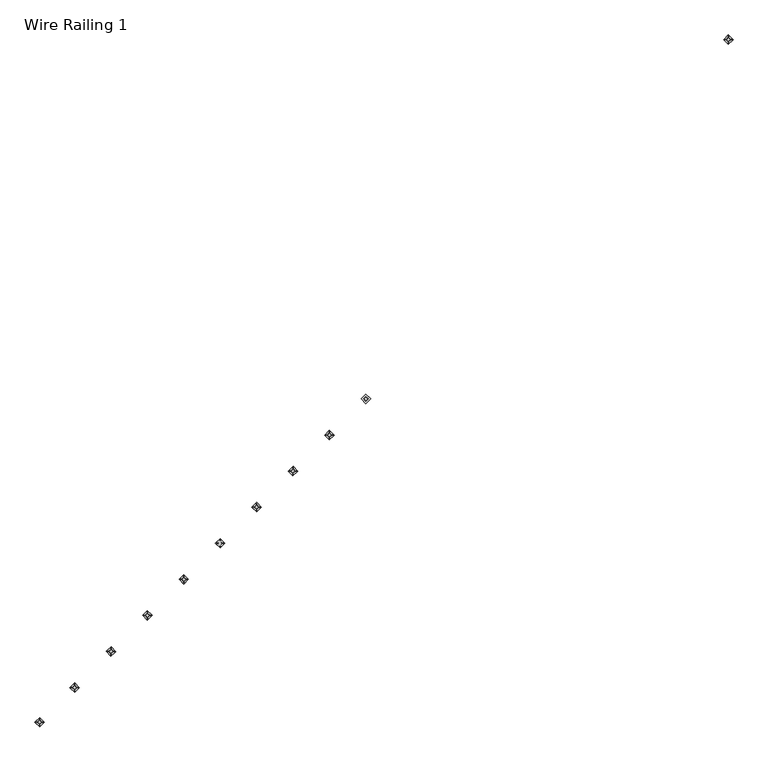
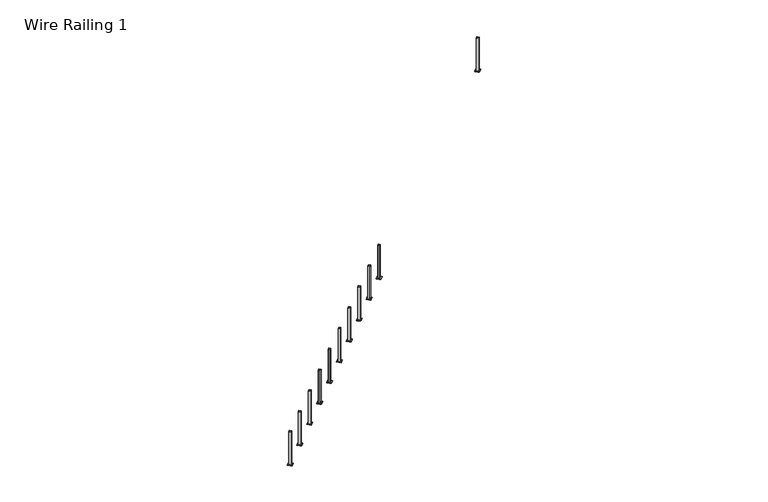
"""IFC4 building model written with IfcOpenShell, lengths in millimetres: railing geometry, Wire Railing 1."""

from ifc_helpers import new_model, si_unit, point, frame, frame_2d, origin, place, context, project, spatial, polyline, circle_curve, trimmed, segment, composite_curve, outline, extrude, source, transform, mapped, element, save


def wire_railing_1_c849696a(model_context):
    return source(origin(), model_context, "Body", "SweptSolid", [
        extrude(outline(polyline([(38725.9551823, 30541.0321501), (38816.1604279, 30630.430213), (38905.5584909, 30540.2249673), (38815.3532452, 30450.8269044), (38725.9551823, 30541.0321501)])), frame((0.0, 0.0, 263956.8), z_axis=(0.0, 0.0, 1.0), x_axis=(1.0, 0.0, 0.0)), (0.0, 0.0, 1.0), 6.35),
        extrude(outline(polyline([(38773.1010508, 30540.8202646), (38815.9485425, 30583.2843445), (38858.4126224, 30540.4368528), (38815.5651307, 30497.9727729), (38773.1010508, 30540.8202646)]), holes=[polyline([(38782.0812162, 30540.7799055), (38815.6054898, 30506.9529383), (38849.4324569, 30540.4772119), (38815.9081833, 30574.3041791), (38782.0812162, 30540.7799055)])]), frame((0.0, 0.0, 263956.8), z_axis=(0.0, 0.0, 1.0), x_axis=(1.0, 0.0, 0.0)), (0.0, 0.0, 1.0), 1047.75),
        extrude(outline(composite_curve([segment(trimmed(circle_curve(frame_2d((38120.0580506, 29788.5739154)), 6.35), [point((38124.5279538, 29784.0636531))], [point((38115.5881475, 29793.0841776))], False, "CARTESIAN"), True, "CONTINUOUS"), segment(trimmed(circle_curve(frame_2d((38120.0580506, 29788.5739154)), 6.35), [point((38115.5881475, 29793.0841776))], [point((38124.5279538, 29784.0636531))], False, "CARTESIAN"), True, "CONTINUOUS")], self_intersect=False)), frame((0.0, 0.0, 263956.8), z_axis=(0.0, 0.0, 1.0), x_axis=(1.0, 0.0, 0.0)), (0.0, 0.0, 1.0), 12.7),
        extrude(outline(composite_curve([segment(trimmed(circle_curve(frame_2d((38057.4794066, 29851.7175873)), 6.35), [point((38061.9493097, 29847.207325))], [point((38053.0095034, 29856.2278496))], False, "CARTESIAN"), True, "CONTINUOUS"), segment(trimmed(circle_curve(frame_2d((38057.4794066, 29851.7175873)), 6.35), [point((38053.0095034, 29856.2278496))], [point((38061.9493097, 29847.207325))], False, "CARTESIAN"), True, "CONTINUOUS")], self_intersect=False)), frame((0.0, 0.0, 263956.8), z_axis=(0.0, 0.0, 1.0), x_axis=(1.0, 0.0, 0.0)), (0.0, 0.0, 1.0), 12.7),
        extrude(outline(composite_curve([segment(trimmed(circle_curve(frame_2d((38183.2017226, 29851.1525594)), 6.35), [point((38187.6716257, 29846.6422971))], [point((38178.7318194, 29855.6628217))], False, "CARTESIAN"), True, "CONTINUOUS"), segment(trimmed(circle_curve(frame_2d((38183.2017226, 29851.1525594)), 6.35), [point((38178.7318194, 29855.6628217))], [point((38187.6716257, 29846.6422971))], False, "CARTESIAN"), True, "CONTINUOUS")], self_intersect=False)), frame((0.0, 0.0, 263956.8), z_axis=(0.0, 0.0, 1.0), x_axis=(1.0, 0.0, 0.0)), (0.0, 0.0, 1.0), 12.7),
        extrude(outline(composite_curve([segment(trimmed(circle_curve(frame_2d((38120.6230785, 29914.2962314)), 6.35), [point((38125.0929817, 29909.7859691))], [point((38116.1531754, 29918.8064936))], False, "CARTESIAN"), True, "CONTINUOUS"), segment(trimmed(circle_curve(frame_2d((38120.6230785, 29914.2962314)), 6.35), [point((38116.1531754, 29918.8064936))], [point((38125.0929817, 29909.7859691))], False, "CARTESIAN"), True, "CONTINUOUS")], self_intersect=False)), frame((0.0, 0.0, 263956.8), z_axis=(0.0, 0.0, 1.0), x_axis=(1.0, 0.0, 0.0)), (0.0, 0.0, 1.0), 12.7),
        extrude(outline(polyline([(38030.5389103, 29851.8386647), (38120.7441559, 29941.2367277), (38210.1422189, 29851.031482), (38119.9369732, 29761.6334191), (38030.5389103, 29851.8386647)])), frame((0.0, 0.0, 263956.8), z_axis=(0.0, 0.0, 1.0), x_axis=(1.0, 0.0, 0.0)), (0.0, 0.0, 1.0), 6.35),
        extrude(outline(polyline([(38077.6847788, 29851.6267793), (38120.5322705, 29894.0908591), (38162.9963504, 29851.2433675), (38120.1488587, 29808.7792876), (38077.6847788, 29851.6267793)]), holes=[polyline([(38086.6649442, 29851.5864201), (38120.1892178, 29817.759453), (38154.0161849, 29851.2837266), (38120.4919113, 29885.1106937), (38086.6649442, 29851.5864201)])]), frame((0.0, 0.0, 263956.8), z_axis=(0.0, 0.0, 1.0), x_axis=(1.0, 0.0, 0.0)), (0.0, 0.0, 1.0), 1047.75),
        extrude(outline(composite_curve([segment(trimmed(circle_curve(frame_2d((37424.6417786, 29099.38043)), 6.35), [point((37429.1116818, 29094.8701677))], [point((37420.1718755, 29103.8906923))], False, "CARTESIAN"), True, "CONTINUOUS"), segment(trimmed(circle_curve(frame_2d((37424.6417786, 29099.38043)), 6.35), [point((37420.1718755, 29103.8906923))], [point((37429.1116818, 29094.8701677))], False, "CARTESIAN"), True, "CONTINUOUS")], self_intersect=False)), frame((0.0, 0.0, 263956.8), z_axis=(0.0, 0.0, 1.0), x_axis=(1.0, 0.0, 0.0)), (0.0, 0.0, 1.0), 12.7),
        extrude(outline(composite_curve([segment(trimmed(circle_curve(frame_2d((37362.0631346, 29162.524102)), 6.35), [point((37366.5330377, 29158.0138397))], [point((37357.5932314, 29167.0343643))], False, "CARTESIAN"), True, "CONTINUOUS"), segment(trimmed(circle_curve(frame_2d((37362.0631346, 29162.524102)), 6.35), [point((37357.5932314, 29167.0343643))], [point((37366.5330377, 29158.0138397))], False, "CARTESIAN"), True, "CONTINUOUS")], self_intersect=False)), frame((0.0, 0.0, 263956.8), z_axis=(0.0, 0.0, 1.0), x_axis=(1.0, 0.0, 0.0)), (0.0, 0.0, 1.0), 12.7),
        extrude(outline(composite_curve([segment(trimmed(circle_curve(frame_2d((37487.7854506, 29161.9590741)), 6.35), [point((37492.2553537, 29157.4488118))], [point((37483.3155474, 29166.4693364))], False, "CARTESIAN"), True, "CONTINUOUS"), segment(trimmed(circle_curve(frame_2d((37487.7854506, 29161.9590741)), 6.35), [point((37483.3155474, 29166.4693364))], [point((37492.2553537, 29157.4488118))], False, "CARTESIAN"), True, "CONTINUOUS")], self_intersect=False)), frame((0.0, 0.0, 263956.8), z_axis=(0.0, 0.0, 1.0), x_axis=(1.0, 0.0, 0.0)), (0.0, 0.0, 1.0), 12.7),
        extrude(outline(composite_curve([segment(trimmed(circle_curve(frame_2d((37425.2068065, 29225.102746)), 6.35), [point((37429.6767097, 29220.5924837))], [point((37420.7369034, 29229.6130083))], False, "CARTESIAN"), True, "CONTINUOUS"), segment(trimmed(circle_curve(frame_2d((37425.2068065, 29225.102746)), 6.35), [point((37420.7369034, 29229.6130083))], [point((37429.6767097, 29220.5924837))], False, "CARTESIAN"), True, "CONTINUOUS")], self_intersect=False)), frame((0.0, 0.0, 263956.8), z_axis=(0.0, 0.0, 1.0), x_axis=(1.0, 0.0, 0.0)), (0.0, 0.0, 1.0), 12.7),
        extrude(outline(polyline([(37335.1226383, 29162.6451794), (37425.3278839, 29252.0432423), (37514.7259469, 29161.8379967), (37424.5207012, 29072.4399337), (37335.1226383, 29162.6451794)])), frame((0.0, 0.0, 263956.8), z_axis=(0.0, 0.0, 1.0), x_axis=(1.0, 0.0, 0.0)), (0.0, 0.0, 1.0), 6.35),
        extrude(outline(polyline([(37382.2685068, 29162.4332939), (37425.1159985, 29204.8973738), (37467.5800784, 29162.0498821), (37424.7325867, 29119.5858022), (37382.2685068, 29162.4332939)]), holes=[polyline([(37391.2486722, 29162.3929348), (37424.7729458, 29128.5659677), (37458.5999129, 29162.0902413), (37425.0756393, 29195.9172084), (37391.2486722, 29162.3929348)])]), frame((0.0, 0.0, 263956.8), z_axis=(0.0, 0.0, 1.0), x_axis=(1.0, 0.0, 0.0)), (0.0, 0.0, 1.0), 1047.75),
        extrude(outline(composite_curve([segment(trimmed(circle_curve(frame_2d((36729.2255066, 28410.1869447)), 6.35), [point((36733.6954098, 28405.6766824))], [point((36724.7556035, 28414.697207))], False, "CARTESIAN"), True, "CONTINUOUS"), segment(trimmed(circle_curve(frame_2d((36729.2255066, 28410.1869447)), 6.35), [point((36724.7556035, 28414.697207))], [point((36733.6954098, 28405.6766824))], False, "CARTESIAN"), True, "CONTINUOUS")], self_intersect=False)), frame((0.0, 0.0, 263956.8), z_axis=(0.0, 0.0, 1.0), x_axis=(1.0, 0.0, 0.0)), (0.0, 0.0, 1.0), 12.7),
        extrude(outline(composite_curve([segment(trimmed(circle_curve(frame_2d((36666.6468626, 28473.3306166)), 6.35), [point((36671.1167657, 28468.8203544))], [point((36662.1769594, 28477.8408789))], False, "CARTESIAN"), True, "CONTINUOUS"), segment(trimmed(circle_curve(frame_2d((36666.6468626, 28473.3306166)), 6.35), [point((36662.1769594, 28477.8408789))], [point((36671.1167657, 28468.8203544))], False, "CARTESIAN"), True, "CONTINUOUS")], self_intersect=False)), frame((0.0, 0.0, 263956.8), z_axis=(0.0, 0.0, 1.0), x_axis=(1.0, 0.0, 0.0)), (0.0, 0.0, 1.0), 12.7),
        extrude(outline(composite_curve([segment(trimmed(circle_curve(frame_2d((36792.3691786, 28472.7655887)), 6.35), [point((36796.8390817, 28468.2553265))], [point((36787.8992754, 28477.275851))], False, "CARTESIAN"), True, "CONTINUOUS"), segment(trimmed(circle_curve(frame_2d((36792.3691786, 28472.7655887)), 6.35), [point((36787.8992754, 28477.275851))], [point((36796.8390817, 28468.2553265))], False, "CARTESIAN"), True, "CONTINUOUS")], self_intersect=False)), frame((0.0, 0.0, 263956.8), z_axis=(0.0, 0.0, 1.0), x_axis=(1.0, 0.0, 0.0)), (0.0, 0.0, 1.0), 12.7),
        extrude(outline(composite_curve([segment(trimmed(circle_curve(frame_2d((36729.7905345, 28535.9092607)), 6.35), [point((36734.2604377, 28531.3989984))], [point((36725.3206314, 28540.419523))], False, "CARTESIAN"), True, "CONTINUOUS"), segment(trimmed(circle_curve(frame_2d((36729.7905345, 28535.9092607)), 6.35), [point((36725.3206314, 28540.419523))], [point((36734.2604377, 28531.3989984))], False, "CARTESIAN"), True, "CONTINUOUS")], self_intersect=False)), frame((0.0, 0.0, 263956.8), z_axis=(0.0, 0.0, 1.0), x_axis=(1.0, 0.0, 0.0)), (0.0, 0.0, 1.0), 12.7),
        extrude(outline(polyline([(36639.7063663, 28473.4516941), (36729.9116119, 28562.849757), (36819.3096749, 28472.6445113), (36729.1044292, 28383.2464484), (36639.7063663, 28473.4516941)])), frame((0.0, 0.0, 263956.8), z_axis=(0.0, 0.0, 1.0), x_axis=(1.0, 0.0, 0.0)), (0.0, 0.0, 1.0), 6.35),
        extrude(outline(polyline([(36686.8522348, 28473.2398086), (36729.6997265, 28515.7038885), (36772.1638064, 28472.8563968), (36729.3163147, 28430.3923169), (36686.8522348, 28473.2398086)]), holes=[polyline([(36695.8324002, 28473.1994495), (36729.3566738, 28439.3724823), (36763.1836409, 28472.8967559), (36729.6593673, 28506.7237231), (36695.8324002, 28473.1994495)])]), frame((0.0, 0.0, 263956.8), z_axis=(0.0, 0.0, 1.0), x_axis=(1.0, 0.0, 0.0)), (0.0, 0.0, 1.0), 1047.75),
        extrude(outline(composite_curve([segment(trimmed(circle_curve(frame_2d((36033.8092346, 27720.9934594)), 6.35), [point((36038.2791378, 27716.4831971))], [point((36029.3393315, 27725.5037216))], False, "CARTESIAN"), True, "CONTINUOUS"), segment(trimmed(circle_curve(frame_2d((36033.8092346, 27720.9934594)), 6.35), [point((36029.3393315, 27725.5037216))], [point((36038.2791378, 27716.4831971))], False, "CARTESIAN"), True, "CONTINUOUS")], self_intersect=False)), frame((0.0, 0.0, 263956.8), z_axis=(0.0, 0.0, 1.0), x_axis=(1.0, 0.0, 0.0)), (0.0, 0.0, 1.0), 12.7),
        extrude(outline(composite_curve([segment(trimmed(circle_curve(frame_2d((35971.2305906, 27784.1371313)), 6.35), [point((35975.7004937, 27779.626869))], [point((35966.7606874, 27788.6473936))], False, "CARTESIAN"), True, "CONTINUOUS"), segment(trimmed(circle_curve(frame_2d((35971.2305906, 27784.1371313)), 6.35), [point((35966.7606874, 27788.6473936))], [point((35975.7004937, 27779.626869))], False, "CARTESIAN"), True, "CONTINUOUS")], self_intersect=False)), frame((0.0, 0.0, 263956.8), z_axis=(0.0, 0.0, 1.0), x_axis=(1.0, 0.0, 0.0)), (0.0, 0.0, 1.0), 12.7),
        extrude(outline(composite_curve([segment(trimmed(circle_curve(frame_2d((36096.9529066, 27783.5721034)), 6.35), [point((36101.4228097, 27779.0618411))], [point((36092.4830034, 27788.0823657))], False, "CARTESIAN"), True, "CONTINUOUS"), segment(trimmed(circle_curve(frame_2d((36096.9529066, 27783.5721034)), 6.35), [point((36092.4830034, 27788.0823657))], [point((36101.4228097, 27779.0618411))], False, "CARTESIAN"), True, "CONTINUOUS")], self_intersect=False)), frame((0.0, 0.0, 263956.8), z_axis=(0.0, 0.0, 1.0), x_axis=(1.0, 0.0, 0.0)), (0.0, 0.0, 1.0), 12.7),
        extrude(outline(composite_curve([segment(trimmed(circle_curve(frame_2d((36034.3742625, 27846.7157754)), 6.35), [point((36038.8441657, 27842.2055131))], [point((36029.9043594, 27851.2260376))], False, "CARTESIAN"), True, "CONTINUOUS"), segment(trimmed(circle_curve(frame_2d((36034.3742625, 27846.7157754)), 6.35), [point((36029.9043594, 27851.2260376))], [point((36038.8441657, 27842.2055131))], False, "CARTESIAN"), True, "CONTINUOUS")], self_intersect=False)), frame((0.0, 0.0, 263956.8), z_axis=(0.0, 0.0, 1.0), x_axis=(1.0, 0.0, 0.0)), (0.0, 0.0, 1.0), 12.7),
        extrude(outline(polyline([(35944.2900943, 27784.2582087), (36034.4953399, 27873.6562717), (36123.8934029, 27783.451026), (36033.6881572, 27694.0529631), (35944.2900943, 27784.2582087)])), frame((0.0, 0.0, 263956.8), z_axis=(0.0, 0.0, 1.0), x_axis=(1.0, 0.0, 0.0)), (0.0, 0.0, 1.0), 6.35),
        extrude(outline(polyline([(35991.4359628, 27784.0463233), (36034.2834545, 27826.5104031), (36076.7475344, 27783.6629115), (36033.9000427, 27741.1988316), (35991.4359628, 27784.0463233)]), holes=[polyline([(36000.4161282, 27784.0059641), (36033.9404018, 27750.178997), (36067.7673689, 27783.7032706), (36034.2430953, 27817.5302377), (36000.4161282, 27784.0059641)])]), frame((0.0, 0.0, 263956.8), z_axis=(0.0, 0.0, 1.0), x_axis=(1.0, 0.0, 0.0)), (0.0, 0.0, 1.0), 1047.75),
        extrude(outline(composite_curve([segment(trimmed(circle_curve(frame_2d((35338.3929626, 27031.799974)), 6.35), [point((35342.8628658, 27027.2897117))], [point((35333.9230595, 27036.3102363))], False, "CARTESIAN"), True, "CONTINUOUS"), segment(trimmed(circle_curve(frame_2d((35338.3929626, 27031.799974)), 6.35), [point((35333.9230595, 27036.3102363))], [point((35342.8628658, 27027.2897117))], False, "CARTESIAN"), True, "CONTINUOUS")], self_intersect=False)), frame((0.0, 0.0, 263956.8), z_axis=(0.0, 0.0, 1.0), x_axis=(1.0, 0.0, 0.0)), (0.0, 0.0, 1.0), 12.7),
        extrude(outline(composite_curve([segment(trimmed(circle_curve(frame_2d((35275.8143186, 27094.943646)), 6.35), [point((35280.2842217, 27090.4333837))], [point((35271.3444154, 27099.4539083))], False, "CARTESIAN"), True, "CONTINUOUS"), segment(trimmed(circle_curve(frame_2d((35275.8143186, 27094.943646)), 6.35), [point((35271.3444154, 27099.4539083))], [point((35280.2842217, 27090.4333837))], False, "CARTESIAN"), True, "CONTINUOUS")], self_intersect=False)), frame((0.0, 0.0, 263956.8), z_axis=(0.0, 0.0, 1.0), x_axis=(1.0, 0.0, 0.0)), (0.0, 0.0, 1.0), 12.7),
        extrude(outline(composite_curve([segment(trimmed(circle_curve(frame_2d((35401.5366346, 27094.3786181)), 6.35), [point((35406.0065377, 27089.8683558))], [point((35397.0667314, 27098.8888804))], False, "CARTESIAN"), True, "CONTINUOUS"), segment(trimmed(circle_curve(frame_2d((35401.5366346, 27094.3786181)), 6.35), [point((35397.0667314, 27098.8888804))], [point((35406.0065377, 27089.8683558))], False, "CARTESIAN"), True, "CONTINUOUS")], self_intersect=False)), frame((0.0, 0.0, 263956.8), z_axis=(0.0, 0.0, 1.0), x_axis=(1.0, 0.0, 0.0)), (0.0, 0.0, 1.0), 12.7),
        extrude(outline(composite_curve([segment(trimmed(circle_curve(frame_2d((35338.9579905, 27157.52229)), 6.35), [point((35343.4278937, 27153.0120277))], [point((35334.4880874, 27162.0325523))], False, "CARTESIAN"), True, "CONTINUOUS"), segment(trimmed(circle_curve(frame_2d((35338.9579905, 27157.52229)), 6.35), [point((35334.4880874, 27162.0325523))], [point((35343.4278937, 27153.0120277))], False, "CARTESIAN"), True, "CONTINUOUS")], self_intersect=False)), frame((0.0, 0.0, 263956.8), z_axis=(0.0, 0.0, 1.0), x_axis=(1.0, 0.0, 0.0)), (0.0, 0.0, 1.0), 12.7),
        extrude(outline(polyline([(35248.8738223, 27095.0647234), (35339.0790679, 27184.4627863), (35428.4771309, 27094.2575407), (35338.2718852, 27004.8594777), (35248.8738223, 27095.0647234)])), frame((0.0, 0.0, 263956.8), z_axis=(0.0, 0.0, 1.0), x_axis=(1.0, 0.0, 0.0)), (0.0, 0.0, 1.0), 6.35),
        extrude(outline(polyline([(35296.0196908, 27094.8528379), (35338.8671825, 27137.3169178), (35381.3312624, 27094.4694261), (35338.4837707, 27052.0053462), (35296.0196908, 27094.8528379)]), holes=[polyline([(35304.9998562, 27094.8124788), (35338.5241298, 27060.9855117), (35372.3510969, 27094.5097853), (35338.8268233, 27128.3367524), (35304.9998562, 27094.8124788)])]), frame((0.0, 0.0, 263956.8), z_axis=(0.0, 0.0, 1.0), x_axis=(1.0, 0.0, 0.0)), (0.0, 0.0, 1.0), 1047.75),
        extrude(outline(composite_curve([segment(trimmed(circle_curve(frame_2d((34642.9766906, 26342.6064887)), 6.35), [point((34647.4465938, 26338.0962264))], [point((34638.5067875, 26347.116751))], False, "CARTESIAN"), True, "CONTINUOUS"), segment(trimmed(circle_curve(frame_2d((34642.9766906, 26342.6064887)), 6.35), [point((34638.5067875, 26347.116751))], [point((34647.4465938, 26338.0962264))], False, "CARTESIAN"), True, "CONTINUOUS")], self_intersect=False)), frame((0.0, 0.0, 263956.8), z_axis=(0.0, 0.0, 1.0), x_axis=(1.0, 0.0, 0.0)), (0.0, 0.0, 1.0), 12.7),
        extrude(outline(composite_curve([segment(trimmed(circle_curve(frame_2d((34580.3980466, 26405.7501606)), 6.35), [point((34584.8679497, 26401.2398984))], [point((34575.9281434, 26410.2604229))], False, "CARTESIAN"), True, "CONTINUOUS"), segment(trimmed(circle_curve(frame_2d((34580.3980466, 26405.7501606)), 6.35), [point((34575.9281434, 26410.2604229))], [point((34584.8679497, 26401.2398984))], False, "CARTESIAN"), True, "CONTINUOUS")], self_intersect=False)), frame((0.0, 0.0, 263956.8), z_axis=(0.0, 0.0, 1.0), x_axis=(1.0, 0.0, 0.0)), (0.0, 0.0, 1.0), 12.7),
        extrude(outline(composite_curve([segment(trimmed(circle_curve(frame_2d((34706.1203626, 26405.1851327)), 6.35), [point((34710.5902657, 26400.6748705))], [point((34701.6504594, 26409.695395))], False, "CARTESIAN"), True, "CONTINUOUS"), segment(trimmed(circle_curve(frame_2d((34706.1203626, 26405.1851327)), 6.35), [point((34701.6504594, 26409.695395))], [point((34710.5902657, 26400.6748705))], False, "CARTESIAN"), True, "CONTINUOUS")], self_intersect=False)), frame((0.0, 0.0, 263956.8), z_axis=(0.0, 0.0, 1.0), x_axis=(1.0, 0.0, 0.0)), (0.0, 0.0, 1.0), 12.7),
        extrude(outline(composite_curve([segment(trimmed(circle_curve(frame_2d((34643.5417185, 26468.3288047)), 6.35), [point((34648.0116217, 26463.8185424))], [point((34639.0718154, 26472.839067))], False, "CARTESIAN"), True, "CONTINUOUS"), segment(trimmed(circle_curve(frame_2d((34643.5417185, 26468.3288047)), 6.35), [point((34639.0718154, 26472.839067))], [point((34648.0116217, 26463.8185424))], False, "CARTESIAN"), True, "CONTINUOUS")], self_intersect=False)), frame((0.0, 0.0, 263956.8), z_axis=(0.0, 0.0, 1.0), x_axis=(1.0, 0.0, 0.0)), (0.0, 0.0, 1.0), 12.7),
        extrude(outline(polyline([(34553.4575503, 26405.8712381), (34643.6627959, 26495.269301), (34733.0608589, 26405.0640553), (34642.8556132, 26315.6659924), (34553.4575503, 26405.8712381)])), frame((0.0, 0.0, 263956.8), z_axis=(0.0, 0.0, 1.0), x_axis=(1.0, 0.0, 0.0)), (0.0, 0.0, 1.0), 6.35),
        extrude(outline(polyline([(34600.6034188, 26405.6593526), (34643.4509105, 26448.1234325), (34685.9149903, 26405.2759408), (34643.0674987, 26362.8118609), (34600.6034188, 26405.6593526)]), holes=[polyline([(34609.5835842, 26405.6189935), (34643.1078578, 26371.7920263), (34676.9348249, 26405.3162999), (34643.4105513, 26439.1432671), (34609.5835842, 26405.6189935)])]), frame((0.0, 0.0, 263956.8), z_axis=(0.0, 0.0, 1.0), x_axis=(1.0, 0.0, 0.0)), (0.0, 0.0, 1.0), 1047.75),
        extrude(outline(composite_curve([segment(trimmed(circle_curve(frame_2d((33947.5604186, 25653.4130034)), 6.35), [point((33952.0303217, 25648.9027411))], [point((33943.0905155, 25657.9232656))], False, "CARTESIAN"), True, "CONTINUOUS"), segment(trimmed(circle_curve(frame_2d((33947.5604186, 25653.4130034)), 6.35), [point((33943.0905155, 25657.9232656))], [point((33952.0303217, 25648.9027411))], False, "CARTESIAN"), True, "CONTINUOUS")], self_intersect=False)), frame((0.0, 0.0, 263956.8), z_axis=(0.0, 0.0, 1.0), x_axis=(1.0, 0.0, 0.0)), (0.0, 0.0, 1.0), 12.7),
        extrude(outline(composite_curve([segment(trimmed(circle_curve(frame_2d((33884.9817745, 25716.5566753)), 6.35), [point((33889.4516777, 25712.046413))], [point((33880.5118714, 25721.0669376))], False, "CARTESIAN"), True, "CONTINUOUS"), segment(trimmed(circle_curve(frame_2d((33884.9817745, 25716.5566753)), 6.35), [point((33880.5118714, 25721.0669376))], [point((33889.4516777, 25712.046413))], False, "CARTESIAN"), True, "CONTINUOUS")], self_intersect=False)), frame((0.0, 0.0, 263956.8), z_axis=(0.0, 0.0, 1.0), x_axis=(1.0, 0.0, 0.0)), (0.0, 0.0, 1.0), 12.7),
        extrude(outline(composite_curve([segment(trimmed(circle_curve(frame_2d((34010.7040906, 25715.9916474)), 6.35), [point((34015.1739937, 25711.4813851))], [point((34006.2341874, 25720.5019097))], False, "CARTESIAN"), True, "CONTINUOUS"), segment(trimmed(circle_curve(frame_2d((34010.7040906, 25715.9916474)), 6.35), [point((34006.2341874, 25720.5019097))], [point((34015.1739937, 25711.4813851))], False, "CARTESIAN"), True, "CONTINUOUS")], self_intersect=False)), frame((0.0, 0.0, 263956.8), z_axis=(0.0, 0.0, 1.0), x_axis=(1.0, 0.0, 0.0)), (0.0, 0.0, 1.0), 12.7),
        extrude(outline(composite_curve([segment(trimmed(circle_curve(frame_2d((33948.1254465, 25779.1353194)), 6.35), [point((33952.5953497, 25774.6250571))], [point((33943.6555434, 25783.6455816))], False, "CARTESIAN"), True, "CONTINUOUS"), segment(trimmed(circle_curve(frame_2d((33948.1254465, 25779.1353194)), 6.35), [point((33943.6555434, 25783.6455816))], [point((33952.5953497, 25774.6250571))], False, "CARTESIAN"), True, "CONTINUOUS")], self_intersect=False)), frame((0.0, 0.0, 263956.8), z_axis=(0.0, 0.0, 1.0), x_axis=(1.0, 0.0, 0.0)), (0.0, 0.0, 1.0), 12.7),
        extrude(outline(polyline([(33858.0412783, 25716.6777527), (33948.2465239, 25806.0758157), (34037.6445869, 25715.87057), (33947.4393412, 25626.4725071), (33858.0412783, 25716.6777527)])), frame((0.0, 0.0, 263956.8), z_axis=(0.0, 0.0, 1.0), x_axis=(1.0, 0.0, 0.0)), (0.0, 0.0, 1.0), 6.35),
        extrude(outline(polyline([(33905.1871468, 25716.4658673), (33948.0346385, 25758.9299472), (33990.4987183, 25716.0824555), (33947.6512267, 25673.6183756), (33905.1871468, 25716.4658673)]), holes=[polyline([(33914.1673122, 25716.4255081), (33947.6915858, 25682.598541), (33981.5185529, 25716.1228146), (33947.9942793, 25749.9497817), (33914.1673122, 25716.4255081)])]), frame((0.0, 0.0, 263956.8), z_axis=(0.0, 0.0, 1.0), x_axis=(1.0, 0.0, 0.0)), (0.0, 0.0, 1.0), 1047.75),
        extrude(outline(composite_curve([segment(trimmed(circle_curve(frame_2d((33252.1441466, 24964.219518)), 6.35), [point((33256.6140497, 24959.7092557))], [point((33247.6742435, 24968.7297803))], False, "CARTESIAN"), True, "CONTINUOUS"), segment(trimmed(circle_curve(frame_2d((33252.1441466, 24964.219518)), 6.35), [point((33247.6742435, 24968.7297803))], [point((33256.6140497, 24959.7092557))], False, "CARTESIAN"), True, "CONTINUOUS")], self_intersect=False)), frame((0.0, 0.0, 263956.8), z_axis=(0.0, 0.0, 1.0), x_axis=(1.0, 0.0, 0.0)), (0.0, 0.0, 1.0), 12.7),
        extrude(outline(composite_curve([segment(trimmed(circle_curve(frame_2d((33189.5655025, 25027.36319)), 6.35), [point((33194.0354057, 25022.8529277))], [point((33185.0955994, 25031.8734523))], False, "CARTESIAN"), True, "CONTINUOUS"), segment(trimmed(circle_curve(frame_2d((33189.5655025, 25027.36319)), 6.35), [point((33185.0955994, 25031.8734523))], [point((33194.0354057, 25022.8529277))], False, "CARTESIAN"), True, "CONTINUOUS")], self_intersect=False)), frame((0.0, 0.0, 263956.8), z_axis=(0.0, 0.0, 1.0), x_axis=(1.0, 0.0, 0.0)), (0.0, 0.0, 1.0), 12.7),
        extrude(outline(composite_curve([segment(trimmed(circle_curve(frame_2d((33315.2878186, 25026.7981621)), 6.35), [point((33319.7577217, 25022.2878998))], [point((33310.8179154, 25031.3084244))], False, "CARTESIAN"), True, "CONTINUOUS"), segment(trimmed(circle_curve(frame_2d((33315.2878186, 25026.7981621)), 6.35), [point((33310.8179154, 25031.3084244))], [point((33319.7577217, 25022.2878998))], False, "CARTESIAN"), True, "CONTINUOUS")], self_intersect=False)), frame((0.0, 0.0, 263956.8), z_axis=(0.0, 0.0, 1.0), x_axis=(1.0, 0.0, 0.0)), (0.0, 0.0, 1.0), 12.7),
        extrude(outline(composite_curve([segment(trimmed(circle_curve(frame_2d((33252.7091745, 25089.941834)), 6.35), [point((33257.1790777, 25085.4315718))], [point((33248.2392714, 25094.4520963))], False, "CARTESIAN"), True, "CONTINUOUS"), segment(trimmed(circle_curve(frame_2d((33252.7091745, 25089.941834)), 6.35), [point((33248.2392714, 25094.4520963))], [point((33257.1790777, 25085.4315718))], False, "CARTESIAN"), True, "CONTINUOUS")], self_intersect=False)), frame((0.0, 0.0, 263956.8), z_axis=(0.0, 0.0, 1.0), x_axis=(1.0, 0.0, 0.0)), (0.0, 0.0, 1.0), 12.7),
        extrude(outline(polyline([(33162.6250063, 25027.4842674), (33252.8302519, 25116.8823303), (33342.2283148, 25026.6770847), (33252.0230692, 24937.2790217), (33162.6250063, 25027.4842674)])), frame((0.0, 0.0, 263956.8), z_axis=(0.0, 0.0, 1.0), x_axis=(1.0, 0.0, 0.0)), (0.0, 0.0, 1.0), 6.35),
        extrude(outline(polyline([(33209.7708748, 25027.2723819), (33252.6183664, 25069.7364618), (33295.0824463, 25026.8889701), (33252.2349547, 24984.4248902), (33209.7708748, 25027.2723819)]), holes=[polyline([(33218.7510402, 25027.2320228), (33252.2753138, 24993.4050557), (33286.1022809, 25026.9293293), (33252.5780073, 25060.7562964), (33218.7510402, 25027.2320228)])]), frame((0.0, 0.0, 263956.8), z_axis=(0.0, 0.0, 1.0), x_axis=(1.0, 0.0, 0.0)), (0.0, 0.0, 1.0), 1047.75),
        extrude(outline(composite_curve([segment(trimmed(circle_curve(frame_2d((45742.575469, 37342.8828351)), 6.35), [point((45747.0453721, 37338.3725729))], [point((45738.1055658, 37347.3930974))], False, "CARTESIAN"), True, "CONTINUOUS"), segment(trimmed(circle_curve(frame_2d((45742.575469, 37342.8828351)), 6.35), [point((45738.1055658, 37347.3930974))], [point((45747.0453721, 37338.3725729))], False, "CARTESIAN"), True, "CONTINUOUS")], self_intersect=False)), frame((0.0, 0.0, 263956.8), z_axis=(0.0, 0.0, 1.0), x_axis=(1.0, 0.0, 0.0)), (0.0, 0.0, 1.0), 12.7),
        extrude(outline(composite_curve([segment(trimmed(circle_curve(frame_2d((45679.9968249, 37406.0265071)), 6.35), [point((45684.466728, 37401.5162448))], [point((45675.5269218, 37410.5367694))], False, "CARTESIAN"), True, "CONTINUOUS"), segment(trimmed(circle_curve(frame_2d((45679.9968249, 37406.0265071)), 6.35), [point((45675.5269218, 37410.5367694))], [point((45684.466728, 37401.5162448))], False, "CARTESIAN"), True, "CONTINUOUS")], self_intersect=False)), frame((0.0, 0.0, 263956.8), z_axis=(0.0, 0.0, 1.0), x_axis=(1.0, 0.0, 0.0)), (0.0, 0.0, 1.0), 12.7),
        extrude(outline(composite_curve([segment(trimmed(circle_curve(frame_2d((45805.7191409, 37405.4614792)), 6.35), [point((45810.1890441, 37400.9512169))], [point((45801.2492378, 37409.9717415))], False, "CARTESIAN"), True, "CONTINUOUS"), segment(trimmed(circle_curve(frame_2d((45805.7191409, 37405.4614792)), 6.35), [point((45801.2492378, 37409.9717415))], [point((45810.1890441, 37400.9512169))], False, "CARTESIAN"), True, "CONTINUOUS")], self_intersect=False)), frame((0.0, 0.0, 263956.8), z_axis=(0.0, 0.0, 1.0), x_axis=(1.0, 0.0, 0.0)), (0.0, 0.0, 1.0), 12.7),
        extrude(outline(composite_curve([segment(trimmed(circle_curve(frame_2d((45743.1404969, 37468.6051512)), 6.35), [point((45747.6104, 37464.0948889))], [point((45738.6705937, 37473.1154134))], False, "CARTESIAN"), True, "CONTINUOUS"), segment(trimmed(circle_curve(frame_2d((45743.1404969, 37468.6051512)), 6.35), [point((45738.6705937, 37473.1154134))], [point((45747.6104, 37464.0948889))], False, "CARTESIAN"), True, "CONTINUOUS")], self_intersect=False)), frame((0.0, 0.0, 263956.8), z_axis=(0.0, 0.0, 1.0), x_axis=(1.0, 0.0, 0.0)), (0.0, 0.0, 1.0), 12.7),
        extrude(outline(polyline([(45653.0563286, 37406.1475845), (45743.2615743, 37495.5456474), (45832.6596372, 37405.3404018), (45742.4543915, 37315.9423388), (45653.0563286, 37406.1475845)])), frame((0.0, 0.0, 263956.8), z_axis=(0.0, 0.0, 1.0), x_axis=(1.0, 0.0, 0.0)), (0.0, 0.0, 1.0), 6.35),
        extrude(outline(polyline([(45700.2021971, 37405.935699), (45743.0496888, 37448.3997789), (45785.5137687, 37405.5522872), (45742.666277, 37363.0882074), (45700.2021971, 37405.935699)]), holes=[polyline([(45709.1823625, 37405.8953399), (45742.7066361, 37372.0683728), (45776.5336033, 37405.5926464), (45743.0093297, 37439.4196135), (45709.1823625, 37405.8953399)])]), frame((0.0, 0.0, 263956.8), z_axis=(0.0, 0.0, 1.0), x_axis=(1.0, 0.0, 0.0)), (0.0, 0.0, 1.0), 1047.75),
        extrude(outline(composite_curve([segment(trimmed(circle_curve(frame_2d((32583.7894483, 24301.8454516)), 6.35), [point((32588.2593514, 24297.3351893))], [point((32579.3195451, 24306.3557139))], False, "CARTESIAN"), True, "CONTINUOUS"), segment(trimmed(circle_curve(frame_2d((32583.7894483, 24301.8454516)), 6.35), [point((32579.3195451, 24306.3557139))], [point((32588.2593514, 24297.3351893))], False, "CARTESIAN"), True, "CONTINUOUS")], self_intersect=False)), frame((0.0, 0.0, 263956.8), z_axis=(0.0, 0.0, 1.0), x_axis=(1.0, 0.0, 0.0)), (0.0, 0.0, 1.0), 12.7),
        extrude(outline(composite_curve([segment(trimmed(circle_curve(frame_2d((32521.2108042, 24364.9891235)), 6.35), [point((32525.6807074, 24360.4788612))], [point((32516.7409011, 24369.4993858))], False, "CARTESIAN"), True, "CONTINUOUS"), segment(trimmed(circle_curve(frame_2d((32521.2108042, 24364.9891235)), 6.35), [point((32516.7409011, 24369.4993858))], [point((32525.6807074, 24360.4788612))], False, "CARTESIAN"), True, "CONTINUOUS")], self_intersect=False)), frame((0.0, 0.0, 263956.8), z_axis=(0.0, 0.0, 1.0), x_axis=(1.0, 0.0, 0.0)), (0.0, 0.0, 1.0), 12.7),
        extrude(outline(composite_curve([segment(trimmed(circle_curve(frame_2d((32646.9331203, 24364.4240956)), 6.35), [point((32651.4030234, 24359.9138333))], [point((32642.4632171, 24368.9343579))], False, "CARTESIAN"), True, "CONTINUOUS"), segment(trimmed(circle_curve(frame_2d((32646.9331203, 24364.4240956)), 6.35), [point((32642.4632171, 24368.9343579))], [point((32651.4030234, 24359.9138333))], False, "CARTESIAN"), True, "CONTINUOUS")], self_intersect=False)), frame((0.0, 0.0, 263956.8), z_axis=(0.0, 0.0, 1.0), x_axis=(1.0, 0.0, 0.0)), (0.0, 0.0, 1.0), 12.7),
        extrude(outline(composite_curve([segment(trimmed(circle_curve(frame_2d((32584.3544762, 24427.5677676)), 6.35), [point((32588.8243793, 24423.0575053))], [point((32579.8845731, 24432.0780299))], False, "CARTESIAN"), True, "CONTINUOUS"), segment(trimmed(circle_curve(frame_2d((32584.3544762, 24427.5677676)), 6.35), [point((32579.8845731, 24432.0780299))], [point((32588.8243793, 24423.0575053))], False, "CARTESIAN"), True, "CONTINUOUS")], self_intersect=False)), frame((0.0, 0.0, 263956.8), z_axis=(0.0, 0.0, 1.0), x_axis=(1.0, 0.0, 0.0)), (0.0, 0.0, 1.0), 12.7),
        extrude(outline(polyline([(32494.270308, 24365.1102009), (32584.4755536, 24454.5082639), (32673.8736165, 24364.3030182), (32583.6683709, 24274.9049553), (32494.270308, 24365.1102009)])), frame((0.0, 0.0, 263956.8), z_axis=(0.0, 0.0, 1.0), x_axis=(1.0, 0.0, 0.0)), (0.0, 0.0, 1.0), 6.35),
        extrude(outline(polyline([(32541.4161765, 24364.8983155), (32584.2636681, 24407.3623954), (32626.727748, 24364.5149037), (32583.8802564, 24322.0508238), (32541.4161765, 24364.8983155)]), holes=[polyline([(32550.3963419, 24364.8579563), (32583.9206155, 24331.0309892), (32617.7475826, 24364.5552628), (32584.223309, 24398.3822299), (32550.3963419, 24364.8579563)])]), frame((0.0, 0.0, 263956.8), z_axis=(0.0, 0.0, 1.0), x_axis=(1.0, 0.0, 0.0)), (0.0, 0.0, 1.0), 1047.75),
    ])


if __name__ == "__main__":
    model = new_model("IFC4")
    model_context = context("Model", 3, world=origin())
    ifc_project = project(units=[si_unit("LENGTHUNIT", "METRE", prefix="MILLI")], contexts=[model_context])
    site = spatial("IfcSite", under=ifc_project)
    building = spatial("IfcBuilding", under=site)
    placement = place(None, origin())
    wire_railing_1_shape = wire_railing_1_c849696a(model_context)
    element("IfcRailing", 1, ObjectType="Wire Railing 1", at=placement, inside=building, context=model_context, shape_type="MappedRepresentation", body=[
        mapped(wire_railing_1_shape, transform((0.0, 0.0, 0.0), x_axis=(1.0, 0.0, 0.0), y_axis=(0.0, 1.0, 0.0), z_axis=(0.0, 0.0, 1.0))),
    ])
    save(model, "model.ifc")

# Revit data of these elements
# Element 1 (IfcRailing, "Wire Railing 1")
#   Materials on its faces: "2 1/2\" X 2 1/2\" ALUM. SQUARE POST (38\" O.C. MAX)", "WIRE RAILING (3\" O.C.)", "ALUM. PLATE TOP RAIL"
# Materials
#   "2 1/2\" X 2 1/2\" ALUM. SQUARE POST (38\" O.C. MAX)": class "Metal", colour RGB 244 244 244, transparency 0, Manufacturer = "Kawneer", URL = "http://www.kawneer.com/kawneer/north_america/en/home.asp", Cost = 0
#   "WIRE RAILING (3\" O.C.)": class "Metal", colour RGB 244 244 244, transparency 0, Manufacturer = "Kawneer", URL = "http://www.kawneer.com/kawneer/north_america/en/home.asp", Cost = 0
#   "ALUM. PLATE TOP RAIL": class "Metal", colour RGB 244 244 244, transparency 0, Manufacturer = "Kawneer", URL = "http://www.kawneer.com/kawneer/north_america/en/home.asp", Cost = 0
